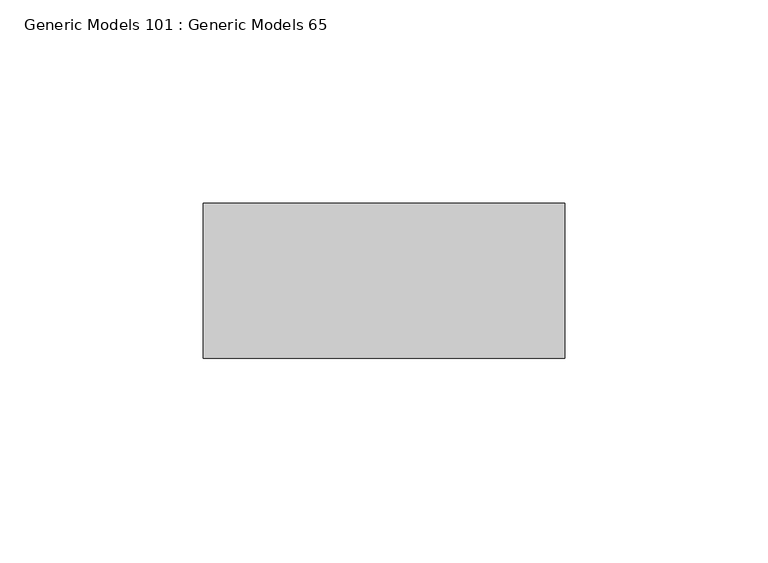
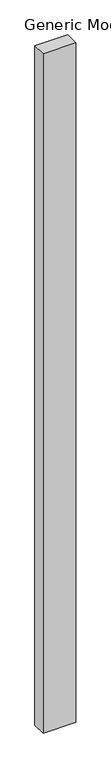
"""IFC4 building model written with IfcOpenShell, lengths in millimetres: proxy geometry, Generic Models 101 : Generic Models 65."""

from ifc_helpers import new_model, si_unit, frame, origin, place, context, project, spatial, polyline, outline, extrude, source, transform, mapped, element, save


def generic_models_101_generic_models_65_cc6b61b5(model_context):
    return source(origin(), model_context, "Body", "SweptSolid", [
        extrude(outline(polyline([(52222.4, 592.1375), (52133.5, 592.1375), (52133.5, 630.2375), (52222.4, 630.2375), (52222.4, 592.1375)])), frame((0.0, 0.0, 3203.178125), z_axis=(0.0, 0.0, 1.0), x_axis=(1.0, 0.0, 0.0)), (0.0, 0.0, 1.0), 1943.1),
    ])


if __name__ == "__main__":
    model = new_model("IFC4")
    model_context = context("Model", 3, world=origin())
    ifc_project = project(units=[si_unit("LENGTHUNIT", "METRE", prefix="MILLI")], contexts=[model_context])
    site = spatial("IfcSite", under=ifc_project)
    building = spatial("IfcBuilding", under=site)
    placement = place(None, origin())
    generic_models_101_generic_models_65_shape = generic_models_101_generic_models_65_cc6b61b5(model_context)
    element("IfcBuildingElementProxy", 1, Name="Generic Models 101 : Generic Models 65", ObjectType="Generic Models 101 : Generic Models 65", at=placement, inside=building, context=model_context, shape_type="MappedRepresentation", body=[
        mapped(generic_models_101_generic_models_65_shape, transform((0.0, 0.0, 0.0), x_axis=(1.0, 0.0, 0.0), y_axis=(0.0, 1.0, 0.0), z_axis=(0.0, 0.0, 1.0))),
    ])
    save(model, "model.ifc")

# Revit data of these elements
# Element 1 (IfcBuildingElementProxy, "Generic Models 101 : Generic Models 65")
#   Materials on its faces: "2X WOOD STUD - SEE 'WALL TAG' & 'LAYER MATERIAL SCHEDULE' FOR SPACING & INSULATION TREATMENT, IF APPLICAPLE"
# Materials
#   "2X WOOD STUD - SEE 'WALL TAG' & 'LAYER MATERIAL SCHEDULE' FOR SPACING & INSULATION TREATMENT, IF APPLICAPLE": class "Wood", colour RGB 234 198 147, transparency 0, Description = "Pinus Echinata", Cost = 0
